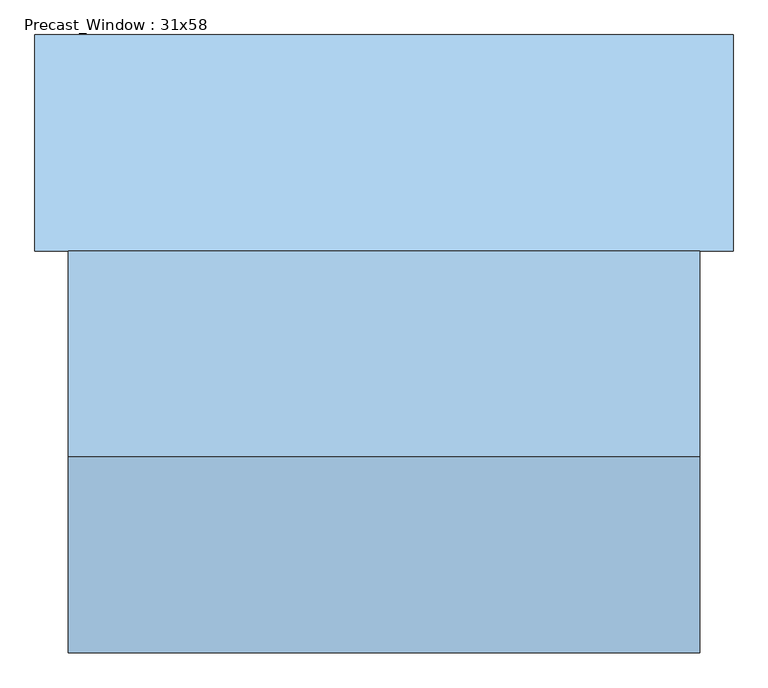
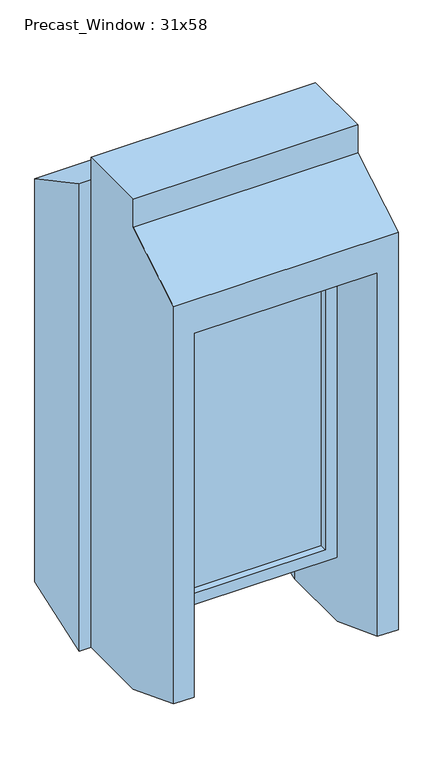
"""IFC4 building model written with IfcOpenShell, lengths in millimetres: window geometry, Precast_Window : 31x58."""

from ifc_helpers import new_model, si_unit, frame, origin, place, context, project, spatial, polyline, outline, extrude, faceted_brep, source, transform, mapped, element, save


def precast_window_31x58_aa46da0b(model_context):
    return source(origin(), model_context, "Body", "SolidModel", [
        extrude(outline(polyline([(342.9, -106.3625), (342.9, -125.4125), (-342.9, -125.4125), (-342.9, -106.3625), (342.9, -106.3625)])), frame((0.0, 0.0, 1066.8), z_axis=(0.0, 0.0, 1.0), x_axis=(1.0, 0.0, 0.0)), (0.0, 0.0, 1.0), 1371.6),
        extrude(outline(polyline([(2489.2, -393.7), (1016.0, -393.7), (1016.0, 393.7), (2489.2, 393.7), (2489.2, -393.7)]), holes=[polyline([(2438.4, -342.9), (2438.4, 342.9), (1066.8, 342.9), (1066.8, -342.9), (2438.4, -342.9)])]), frame((0.0, -157.1625, 0.0), z_axis=(0.0, 1.0, 0.0), x_axis=(0.0, 0.0, 1.0)), (0.0, 0.0, 1.0), 101.6),
        faceted_brep([(482.6, -457.2, 838.2), (482.6, -157.1625, 723.9), (482.6, 157.1625, 723.9), (482.6, 157.1625, 2946.4), (482.6, -157.1625, 2946.4), (482.6, -157.1625, 2819.4), (482.6, -457.2, 2641.6), (393.7, 157.1625, 723.9), (393.7, 157.1625, 2489.2), (-393.7, 157.1625, 2489.2), (-393.7, 157.1625, 723.9), (-482.6, 157.1625, 723.9), (-482.6, 157.1625, 2946.4), (393.7, -457.2, 2489.2), (393.7, -457.2, 838.2), (-482.6, -457.2, 2641.6), (-482.6, -457.2, 838.2), (-393.7, -457.2, 838.2), (-393.7, -457.2, 2489.2), (393.7, -157.1625, 723.9), (-482.6, -157.1625, 2819.4), (-482.6, -157.1625, 2946.4), (-482.6, -157.1625, 723.9), (-393.7, -157.1625, 723.9)], [[[0, 1, 2, 3, 4, 5, 6]], [[7, 8, 9, 10, 11, 12, 3, 2]], [[13, 14, 0, 6, 15, 16, 17, 18]], [[8, 7, 19, 14, 13]], [[16, 15, 20, 21, 12, 11, 22]], [[18, 17, 23, 10, 9]], [[8, 13, 18, 9]], [[4, 3, 12, 21]], [[5, 4, 21, 20]], [[6, 5, 20, 15]], [[1, 0, 14, 19]], [[2, 1, 19, 7]], [[10, 23, 22, 11]], [[23, 17, 16, 22]]]),
        faceted_brep([(533.4, 157.1625, 723.9), (533.4, 487.3625, 838.2), (533.4, 487.3625, 2667.0), (533.4, 157.1625, 2844.8), (393.7, 157.1625, 723.9), (393.7, 487.3625, 838.2), (393.7, 487.3625, 2489.2), (-393.7, 487.3625, 2489.2), (-393.7, 487.3625, 838.2), (-533.4, 487.3625, 838.2), (-533.4, 487.3625, 2667.0), (393.7, 157.1625, 2489.2), (-533.4, 157.1625, 2844.8), (-533.4, 157.1625, 723.9), (-393.7, 157.1625, 723.9), (-393.7, 157.1625, 2489.2)], [[[0, 1, 2, 3]], [[1, 0, 4, 5]], [[5, 6, 7, 8, 9, 10, 2, 1]], [[11, 4, 0, 3, 12, 13, 14, 15]], [[6, 5, 4, 11]], [[13, 12, 10, 9]], [[8, 14, 13, 9]], [[15, 14, 8, 7]], [[3, 2, 10, 12]], [[6, 11, 15, 7]]]),
    ])


if __name__ == "__main__":
    model = new_model("IFC4")
    model_context = context("Model", 3, world=origin())
    ifc_project = project(units=[si_unit("LENGTHUNIT", "METRE", prefix="MILLI")], contexts=[model_context])
    site = spatial("IfcSite", under=ifc_project)
    building = spatial("IfcBuilding", under=site)
    placement = place(None, origin())
    precast_window_31x58_shape = precast_window_31x58_aa46da0b(model_context)
    element("IfcWindow", 1, ObjectType="Precast_Window : 31x58", at=placement, inside=building, context=model_context, shape_type="MappedRepresentation", body=[
        mapped(precast_window_31x58_shape, transform((0.0, 0.0, 0.0), x_axis=(1.0, 0.0, 0.0), y_axis=(0.0, 1.0, 0.0), z_axis=(0.0, 0.0, 1.0))),
    ])
    save(model, "model.ifc")

# Revit data of these elements
# Type "Precast_Window : 31x58"
#   Type Mark = "24"
#   Analytic Construction = "<None>"
#   Height = 4' - 10"
#   Frame Width = 0' - 2"
#   Default Sill Height = 4' - 0"
#   Width = 2' - 7"
#   Precast Material = Stucco - Plaster Cement - Taupe
#   Frame Material = Metal Trim
#   Wall Closure = (empty or 0)
# Element 1 (IfcWindow, "Precast_Window : 31x58")
#   Materials on its faces: "Stucco - Plaster Cement - Taupe", "Metal Trim", "Glass"
# Materials
#   "Stucco - Plaster Cement - Taupe": class "Generic", colour RGB 137 123 107, transparency 0, Description = "Gypsum Wall Board", Cost = 0
#   "Metal Trim": class "Wood", colour RGB 151 137 121, transparency 0, Cost = 0
#   "Glass": class "Glass", colour RGB 218 227 224, transparency 0.85, Description = "Soda Lime Glass", Cost = 0
